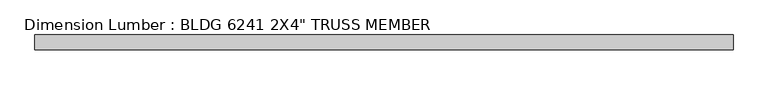
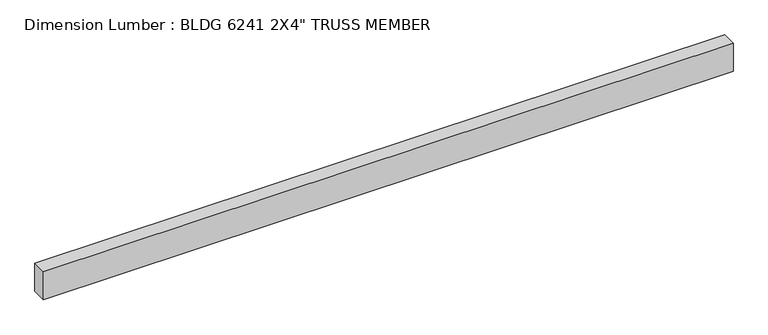
"""IFC4 building model written with IfcOpenShell, lengths in millimetres: beam geometry."""

from ifc_helpers import new_model, si_unit, frame, origin, place, context, project, spatial, polyline, outline, extrude, source, transform, mapped, element, save


def beam_af15350c(model_context):
    return source(origin(), model_context, "Body", "SweptSolid", [
        extrude(outline(polyline([(1181.1, 25.4), (1181.1, -25.4), (-1181.1, -25.4), (-1181.1, 25.4), (1181.1, 25.4)])), frame((0.0, 0.0, -50.8), z_axis=(0.0, 0.0, 1.0), x_axis=(1.0, 0.0, 0.0)), (0.0, 0.0, 1.0), 101.6),
    ])


if __name__ == "__main__":
    model = new_model("IFC4")
    model_context = context("Model", 3, world=origin())
    ifc_project = project(units=[si_unit("LENGTHUNIT", "METRE", prefix="MILLI")], contexts=[model_context])
    site = spatial("IfcSite", under=ifc_project)
    building = spatial("IfcBuilding", under=site)
    placement = place(None, origin())
    beam_shape = beam_af15350c(model_context)
    element("IfcBeam", 1, ObjectType="Dimension Lumber : BLDG 6241 2X4\" TRUSS MEMBER", at=placement, inside=building, context=model_context, shape_type="MappedRepresentation", body=[
        mapped(beam_shape, transform((0.0, 0.0, 0.0), x_axis=(1.0, 0.0, 0.0), y_axis=(0.0, 1.0, 0.0), z_axis=(0.0, 0.0, 1.0))),
    ])
    save(model, "model.ifc")

# Revit data of these elements
# Type "Dimension Lumber : BLDG 6241 2X4\" TRUSS MEMBER"
#   Assembly Code = "B10"
#   A = 0.273472 SF
#   Length [instance default] = 5' - 0"
#   b = 0' - 2"
#   d = 0' - 4"
#   Structural Material [instance default] = Softwood, Lumber
# Element 1 (IfcBeam, "Dimension Lumber : BLDG 6241 2X4\" TRUSS MEMBER")
#   Materials on its faces: "Softwood, Lumber"
# Materials
#   "Softwood, Lumber": class "Wood", colour RGB 223 192 134, transparency 0, Description = "Pinus Echinata", Cost = 0
